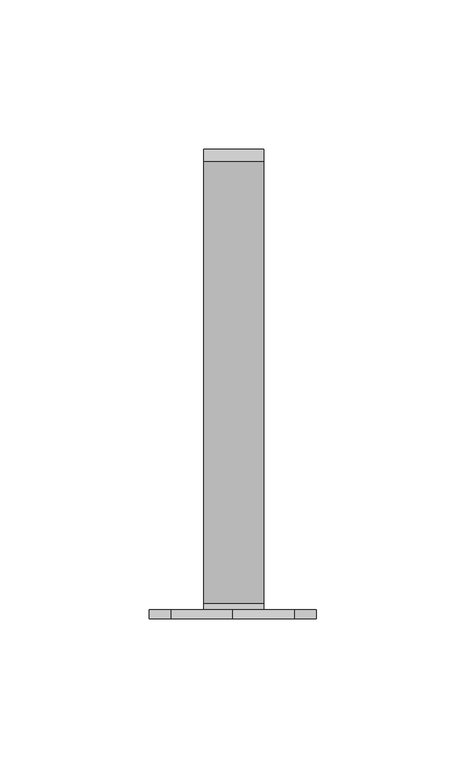
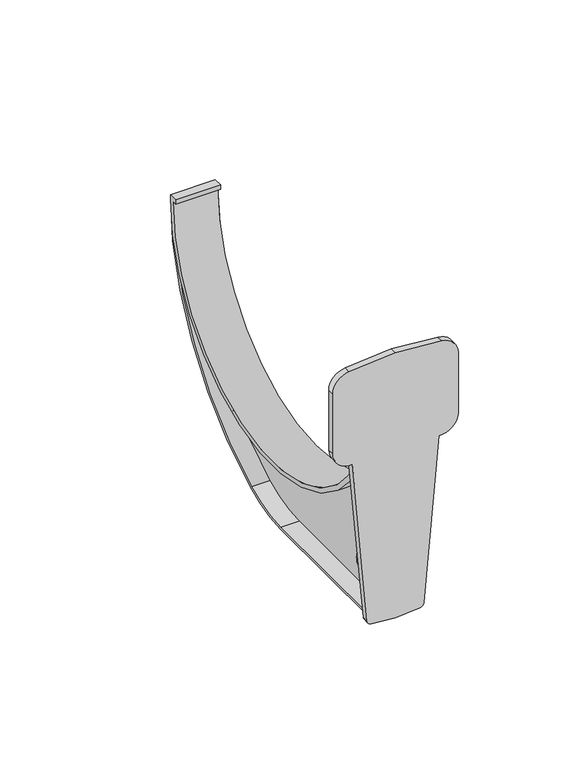
"""IFC4 building model written with IfcOpenShell, lengths in millimetres: proxy geometry, ➾ Кронштейн пластиковый с удлинителем боковым : ➾ Кронштейн пластиковый с удлинителем боковым."""

from ifc_helpers import new_model, si_unit, point, frame, frame_2d, origin, place, context, project, spatial, polyline, circle_curve, trimmed, segment, composite_curve, outline, extrude, source, transform, mapped, element, save
from ifc_brep_helpers import plane_surface, cylinder_surface, revolved_surface, advanced_brep


def generic_models_82e1240d(model_context):
    return source(origin(), model_context, "Body", "SolidModel", [
        advanced_brep(
        [(10.0, 78.1, 0.0), (10.0, 78.1, 2.0), (10.0, 74.055208, 2.0), (10.0, 74.055208, 0.0), (10.0, 76.1, 0.0), (10.0, -76.1, 0.0), (10.0, -76.1, -17.5613211), (-10.0, -76.1, 0.0), (-10.0, 76.1, 0.0), (-10.0, 74.055208, 0.0), (-10.0, 74.055208, 2.0), (-10.0, 78.1, 2.0), (-10.0, 78.1, 0.0), (-10.0, -76.1, -17.5613211), (1.5, -76.1, -17.5613211), (1.5, 71.6158231, -31.1574048), (-1.5, 71.6158231, -31.1574048), (-1.5, -76.1, -17.5613211), (1.5, 76.1, 0.0), (-1.5, 76.1, 0.0), (-1.5, -76.1, 0.0), (1.5, -76.1, 0.0), (1.5, -76.1, -104.0), (1.5, -7.1341862, -104.0), (1.5, 15.3939056, -98.6372612), (1.5, -56.130388, -98.4344464), (1.5, -70.3490278, -98.4344464), (1.5, -70.3490278, -76.8934543), (1.5, -66.9911788, -75.5025877), (1.5, -52.5948541, -89.8989125), (-1.5, 15.3939056, -98.6372612), (-1.5, -7.1341862, -104.0), (-1.5, -76.1, -104.0), (-1.5, -70.3490278, -98.4344464), (-1.5, -56.130388, -98.4344464), (-1.5, -52.5948541, -89.8989125), (-1.5, -66.9911788, -75.5025877), (-1.5, -70.3490278, -76.8934543), (-11.1198282, -79.1, -104.5534176), (-0.2916415, -79.1, -105.5007612), (10.5365453, -79.1, -104.5534176), (12.3546233, -79.1, -102.7353397), (19.0268291, -79.1, -26.4716782), (27.7083585, -79.1, -18.5007612), (27.7083585, -79.1, 9.7189069), (20.4056045, -79.1, 17.6884644), (-0.2807205, -79.1, 19.4982834), (-20.9881575, -79.1, 17.6885282), (-28.2916415, -79.1, 9.7189069), (-28.2916415, -79.1, -18.5007612), (-19.610112, -79.1, -26.4716782), (-12.9379062, -79.1, -102.7353397), (-11.1198282, -76.1, -104.5534176), (-12.9379062, -76.1, -102.7353397), (-19.610112, -76.1, -26.4716782), (-28.2916415, -76.1, -18.5007612), (-28.2916415, -76.1, 9.7189069), (-20.9881575, -76.1, 17.6885283), (-0.2807205, -76.1, 19.4982834), (20.4056045, -76.1, 17.6884644), (27.7083585, -76.1, 9.7189069), (27.7083585, -76.1, -18.5007612), (19.0268291, -76.1, -26.4716782), (12.3546233, -76.1, -102.7353397), (10.5365453, -76.1, -104.5534176), (-0.2916415, -76.1, -105.5007612), (10.0, -76.1, 2.0), (-10.0, -76.1, 2.0), (-10.0, -74.1, 2.0), (10.0, -74.1, 2.0), (-10.0, -74.1, 0.0), (10.0, -74.1, 0.0)],
        [
            (0, 1),
            (1, 2),
            (2, 3),
            (3, 4),
            (4, 5, circle_curve(frame((10.0, 0.0, 0.0), z_axis=(-1.0, 0.0, 0.0), x_axis=(0.0, 1.0, 0.0)), 76.1)),
            (5, 6),
            (6, 0, circle_curve(frame((10.0, 0.0, 0.0), z_axis=(1.0, 0.0, 0.0), x_axis=(0.0, 1.0, 0.0)), 78.1)),
            (7, 8, circle_curve(frame((-10.0, 0.0, 0.0), z_axis=(1.0, 0.0, 0.0), x_axis=(0.0, 1.0, 0.0)), 76.1)),
            (8, 9),
            (9, 10),
            (10, 11),
            (11, 12),
            (12, 13, circle_curve(frame((-10.0, 0.0, 0.0), z_axis=(-1.0, 0.0, 0.0), x_axis=(0.0, 1.0, 0.0)), 78.1)),
            (13, 7),
            (12, 0),
            (6, 14),
            (14, 15, circle_curve(frame((1.5, 0.0, 0.0), z_axis=(1.0, 0.0, 0.0), x_axis=(0.0, 1.0, 0.0)), 78.1)),
            (15, 16),
            (16, 17, circle_curve(frame((-1.5, 0.0, 0.0), z_axis=(-1.0, 0.0, 0.0), x_axis=(0.0, 1.0, 0.0)), 78.1)),
            (17, 13),
            (4, 18),
            (18, 19),
            (19, 8),
            (7, 20),
            (20, 21),
            (21, 5),
            (22, 23),
            (23, 24, circle_curve(frame((1.5, -7.1341862, -54.0), z_axis=(1.0, 0.0, 0.0), x_axis=(0.0, 1.0, 0.0)), 50.0)),
            (24, 15, circle_curve(frame((1.5, -34.3875821, 0.0), z_axis=(1.0, 0.0, 0.0), x_axis=(0.0, 1.0, 0.0)), 110.4875821)),
            (14, 22),
            (25, 26),
            (26, 27),
            (27, 28, circle_curve(frame((1.5, -68.3820454, -76.8934543), z_axis=(-1.0, 0.0, 0.0), x_axis=(0.0, 1.0, 0.0)), 1.9669824)),
            (28, 29),
            (29, 25, circle_curve(frame((1.5, -56.130388, -93.4344464), z_axis=(-1.0, 0.0, 0.0), x_axis=(0.0, 1.0, 0.0)), 5.0)),
            (30, 31, circle_curve(frame((-1.5, -7.1341862, -54.0), z_axis=(-1.0, 0.0, 0.0), x_axis=(0.0, 1.0, 0.0)), 50.0)),
            (31, 32),
            (32, 17),
            (16, 30, circle_curve(frame((-1.5, -34.3875821, 0.0), z_axis=(-1.0, 0.0, 0.0), x_axis=(0.0, 1.0, 0.0)), 110.4875821)),
            (33, 34),
            (34, 35, circle_curve(frame((-1.5, -56.130388, -93.4344464), z_axis=(1.0, 0.0, 0.0), x_axis=(0.0, 1.0, 0.0)), 5.0)),
            (35, 36),
            (36, 37, circle_curve(frame((-1.5, -68.3820454, -76.8934543), z_axis=(1.0, 0.0, 0.0), x_axis=(0.0, 1.0, 0.0)), 1.9669824)),
            (37, 33),
            (22, 32),
            (31, 23),
            (30, 24),
            (38, 39),
            (39, 40),
            (40, 41, circle_curve(frame((10.3622339, -79.1, -102.5610282), z_axis=(0.0, -1.0, 0.0), x_axis=(1.0, 0.0, 0.0)), 2.0)),
            (41, 42),
            (42, 43, circle_curve(frame((19.7083585, -79.1, -18.5007612), z_axis=(0.0, -1.0, 0.0), x_axis=(1.0, 0.0, 0.0)), 8.0)),
            (43, 44),
            (44, 45, circle_curve(frame((19.7083585, -79.1, 9.7189069), z_axis=(0.0, -1.0, 0.0), x_axis=(1.0, 0.0, 0.0)), 8.0)),
            (45, 46),
            (46, 47),
            (47, 48, circle_curve(frame((-20.2916415, -79.1, 9.7189069), z_axis=(0.0, -1.0, 0.0), x_axis=(1.0, 0.0, 0.0)), 8.0)),
            (48, 49),
            (49, 50, circle_curve(frame((-20.2916415, -79.1, -18.5007612), z_axis=(0.0, -1.0, 0.0), x_axis=(1.0, 0.0, 0.0)), 8.0)),
            (50, 51),
            (51, 38, circle_curve(frame((-10.9455168, -79.1, -102.5610282), z_axis=(0.0, -1.0, 0.0), x_axis=(1.0, 0.0, 0.0)), 2.0)),
            (52, 53, circle_curve(frame((-10.9455168, -76.1, -102.5610282), z_axis=(0.0, 1.0, 0.0), x_axis=(1.0, 0.0, 0.0)), 2.0)),
            (53, 54),
            (54, 55, circle_curve(frame((-20.2916415, -76.1, -18.5007612), z_axis=(0.0, 1.0, 0.0), x_axis=(1.0, 0.0, 0.0)), 8.0)),
            (55, 56),
            (56, 57, circle_curve(frame((-20.2916415, -76.1, 9.7189069), z_axis=(0.0, 1.0, 0.0), x_axis=(1.0, 0.0, 0.0)), 8.0)),
            (57, 58),
            (58, 59),
            (59, 60, circle_curve(frame((19.7083585, -76.1, 9.7189069), z_axis=(0.0, 1.0, 0.0), x_axis=(1.0, 0.0, 0.0)), 8.0)),
            (60, 61),
            (61, 62, circle_curve(frame((19.7083585, -76.1, -18.5007612), z_axis=(0.0, 1.0, 0.0), x_axis=(1.0, 0.0, 0.0)), 8.0)),
            (62, 63),
            (63, 64, circle_curve(frame((10.3622339, -76.1, -102.5610282), z_axis=(0.0, 1.0, 0.0), x_axis=(1.0, 0.0, 0.0)), 2.0)),
            (64, 65),
            (65, 52),
            (5, 66),
            (66, 67),
            (67, 7),
            (38, 52),
            (65, 39),
            (64, 40),
            (63, 41),
            (62, 42),
            (61, 43),
            (60, 44),
            (59, 45),
            (58, 46),
            (57, 47),
            (56, 48),
            (55, 49),
            (54, 50),
            (53, 51),
            (33, 26),
            (25, 34),
            (35, 29),
            (28, 36),
            (37, 27),
            (68, 67),
            (66, 69),
            (69, 68),
            (70, 71),
            (71, 5),
            (7, 70),
            (68, 70),
            (71, 69),
            (11, 1),
            (10, 2),
            (9, 3),
        ],
        [
            plane_surface(frame((10.0, -76.1, 0.0), z_axis=(1.0, 0.0, 0.0), x_axis=(0.0, -1.0, 0.0))),
            plane_surface(frame((-10.0, -76.1, 0.0), z_axis=(-1.0, 0.0, 0.0), x_axis=(0.0, 1.0, 0.0))),
            cylinder_surface(frame((-10.0, 0.0, 0.0), z_axis=(1.0, 0.0, 0.0), x_axis=(0.0, 1.0, 0.0)), 78.1),
            revolved_surface(polyline([(-10.0, 76.1, 0.0), (10.0, 76.1, 0.0)]), (-10.0, 0.0, 0.0), (-1.0, 0.0, 0.0)),
            plane_surface(frame((1.5, 76.1, 0.0), z_axis=(1.0, 0.0, 0.0), x_axis=(0.0, 0.0, -1.0))),
            plane_surface(frame((-1.5, 76.1, 0.0), z_axis=(-1.0, 0.0, 0.0), x_axis=(0.0, 0.0, 1.0))),
            plane_surface(frame((1.5, -76.1, -104.0), z_axis=(0.0, 0.0, -1.0), x_axis=(-1.0, 0.0, 0.0))),
            cylinder_surface(frame((-1.5, -7.1341862, -54.0), z_axis=(1.0, 0.0, 0.0), x_axis=(0.0, 1.0, 0.0)), 50.0),
            cylinder_surface(frame((-1.5, -34.3875821, 0.0), z_axis=(1.0, 0.0, 0.0), x_axis=(0.0, 1.0, 0.0)), 110.4875821),
            plane_surface(frame((-11.1198282, -79.1, -104.5534176), z_axis=(0.0, -1.0000000000000002, 0.0), x_axis=(0.9961946980917458, 0.0, -0.08715574274765676))),
            plane_surface(frame((-11.1198282, -76.1, -104.5534176), z_axis=(0.0, 1.0000000000000002, 0.0), x_axis=(-0.9961946980917458, 0.0, 0.08715574274765676))),
            plane_surface(frame((-11.1198282, -79.1, -104.5534176), z_axis=(-0.08715574274765676, 0.0, -0.9961946980917458), x_axis=(0.0, 1.0, 0.0))),
            plane_surface(frame((-0.2916415, -79.1, -105.5007612), z_axis=(0.0871557427476553, 0.0, -0.9961946980917459), x_axis=(0.0, 1.0, 0.0))),
            cylinder_surface(frame((10.3622339, -76.1, -102.5610282), z_axis=(0.0, -1.0, 0.0), x_axis=(1.0, 0.0, 0.0)), 2.0),
            plane_surface(frame((12.3546233, -79.1, -102.7353397), z_axis=(0.9961946980917455, 0.0, -0.08715574274765876), x_axis=(0.0, 1.0, 0.0))),
            cylinder_surface(frame((19.7083585, -76.1, -18.5007612), z_axis=(0.0, -1.0, 0.0), x_axis=(1.0, 0.0, 0.0)), 8.0),
            plane_surface(frame((27.7083585, -79.1, -18.5007612), z_axis=(1.0, 0.0, 0.0), x_axis=(0.0, 1.0, 0.0))),
            cylinder_surface(frame((19.7083585, -76.1, 9.7189069), z_axis=(0.0, -1.0, 0.0), x_axis=(1.0, 0.0, 0.0)), 8.0),
            plane_surface(frame((20.4056045, -79.1, 17.6884644), z_axis=(0.08715574274766355, 0.0, 0.9961946980917451), x_axis=(0.0, 1.0, 0.0))),
            plane_surface(frame((-0.2807205, -79.1, 19.4982834), z_axis=(-0.08706451221038128, 0.0, 0.9962026755201817), x_axis=(0.0, 1.0, 0.0))),
            cylinder_surface(frame((-20.2916415, -76.1, 9.7189069), z_axis=(0.0, -1.0, 0.0), x_axis=(1.0, 0.0, 0.0)), 8.0),
            plane_surface(frame((-28.2916415, -79.1, 9.7189069), z_axis=(-1.0, 0.0, 0.0), x_axis=(0.0, 1.0, 0.0))),
            cylinder_surface(frame((-20.2916415, -76.1, -18.5007612), z_axis=(0.0, -1.0, 0.0), x_axis=(1.0, 0.0, 0.0)), 8.0),
            plane_surface(frame((-19.610112, -79.1, -26.4716782), z_axis=(-0.9961946980917457, 0.0, -0.08715574274765732), x_axis=(0.0, 1.0, 0.0))),
            cylinder_surface(frame((-10.9455168, -76.1, -102.5610282), z_axis=(0.0, -1.0, 0.0), x_axis=(1.0, 0.0, 0.0)), 2.0),
            plane_surface(frame((10.0, -70.3490278, -98.4344464), z_axis=(0.0, 0.0, 1.0), x_axis=(-1.0, 0.0, 0.0))),
            plane_surface(frame((10.0, -52.5948541, -89.8989125), z_axis=(0.0, -0.7071067811865492, -0.7071067811865459), x_axis=(-1.0, 0.0, 0.0))),
            plane_surface(frame((10.0, -70.3490278, -76.8934543), z_axis=(0.0, 1.0, 0.0), x_axis=(-1.0, 0.0, 0.0))),
            revolved_surface(polyline([(1.5, -51.130388, -93.4344464), (-1.5, -51.130388, -93.4344464)]), (-10.0, -56.130388, -93.4344464), (1.0, 0.0, 0.0)),
            revolved_surface(polyline([(1.5, -66.41506299999999, -76.8934543), (-1.5, -66.41506299999999, -76.8934543)]), (-10.0, -68.3820454, -76.8934543), (1.0, 0.0, 0.0)),
            plane_surface(frame((-10.0, -76.1, 2.0), z_axis=(0.0, 0.0, 1.0), x_axis=(0.0, -1.0, 0.0))),
            plane_surface(frame((-10.0, -76.1, 0.0), z_axis=(0.0, 0.0, -1.0), x_axis=(0.0, 1.0, 0.0))),
            plane_surface(frame((-10.0, -74.1, 2.0), z_axis=(-1.0, 0.0, 0.0), x_axis=(0.0, 0.0, -1.0))),
            plane_surface(frame((10.0, -76.1, 2.0), z_axis=(1.0, 0.0, 0.0), x_axis=(0.0, 0.0, -1.0))),
            plane_surface(frame((10.0, -74.1, 2.0), z_axis=(0.0, 1.0, 0.0), x_axis=(0.0, 0.0, -1.0))),
            plane_surface(frame((10.0, 78.1, 0.0), z_axis=(0.0, 1.0, 0.0), x_axis=(-1.0, 0.0, 0.0))),
            plane_surface(frame((10.0, 78.1, 2.0), z_axis=(0.0, 0.0, 1.0), x_axis=(-1.0, 0.0, 0.0))),
            plane_surface(frame((10.0, 74.055208, 2.0), z_axis=(0.0, -1.0, 0.0), x_axis=(-1.0, 0.0, 0.0))),
            plane_surface(frame((10.0, 74.055208, 0.0), z_axis=(0.0, 0.0, -1.0), x_axis=(-1.0, 0.0, 0.0))),
        ],
        [
            (0, [[1, 2, 3, 4, 5, 6, 7]]),
            (1, [[8, 9, 10, 11, 12, 13, 14]]),
            (2, [[15, -7, 16, 17, 18, 19, 20, -13]]),
            (3, [[-5, 21, 22, 23, -8, 24, 25, 26]]),
            (4, [[27, 28, 29, -17, 30], [31, 32, 33, 34, 35]]),
            (5, [[36, 37, 38, -19, 39], [40, 41, 42, 43, 44]]),
            (6, [[-27, 45, -37, 46]]),
            (7, [[-28, -46, -36, 47]]),
            (8, [[-47, -39, -18, -29]]),
            (9, [[48, 49, 50, 51, 52, 53, 54, 55, 56, 57, 58, 59, 60, 61]]),
            (10, [[62, 63, 64, 65, 66, 67, 68, 69, 70, 71, 72, 73, 74, 75], [-6, 76, 77, 78, -14, -20, -38, -45, -30, -16]]),
            (11, [[-48, 79, -75, 80]]),
            (12, [[-49, -80, -74, 81]]),
            (13, [[-50, -81, -73, 82]]),
            (14, [[-51, -82, -72, 83]]),
            (15, [[-52, -83, -71, 84]]),
            (16, [[-53, -84, -70, 85]]),
            (17, [[-54, -85, -69, 86]]),
            (18, [[-55, -86, -68, 87]]),
            (19, [[-56, -87, -67, 88]]),
            (20, [[-57, -88, -66, 89]]),
            (21, [[-58, -89, -65, 90]]),
            (22, [[-59, -90, -64, 91]]),
            (23, [[-60, -91, -63, 92]]),
            (24, [[-61, -92, -62, -79]]),
            (25, [[93, -31, 94, -40]]),
            (26, [[95, -34, 96, -42]]),
            (27, [[-93, -44, 97, -32]]),
            (28, [[-95, -41, -94, -35]]),
            (29, [[-97, -43, -96, -33]]),
            (30, [[98, -77, 99, 100]]),
            (31, [[101, 102, -26, -25, -24, 103]]),
            (32, [[-98, 104, -103, -78]]),
            (33, [[-99, -76, -102, 105]]),
            (34, [[-100, -105, -101, -104]]),
            (35, [[-1, -15, -12, 106]]),
            (36, [[-2, -106, -11, 107]]),
            (37, [[-3, -107, -10, 108]]),
            (38, [[-4, -108, -9, -23, -22, -21]]),
        ],
    ),
        extrude(outline(composite_curve([segment(trimmed(circle_curve(frame_2d((-7.1341862, -53.026974)), 50.0), [point((-7.1341862, -103.026974))], [point((15.3939056, -97.6642352))], True, "CARTESIAN"), True, "CONTINUOUS"), segment(trimmed(circle_curve(frame_2d((-34.3875821, 0.973026)), 110.4875821), [point((15.3939056, -97.6642352))], [point((76.0957154, 0.0))], True, "CARTESIAN"), True, "CONTINUOUS"), segment(polyline([(76.0957154, 0.0), (74.055208, 0.0), (74.055208, 2.0), (78.1, 2.0)]), True, "CONTINUOUS"), segment(trimmed(circle_curve(frame_2d((-34.3875821, 2.0)), 112.4875821), [point((78.1, 2.0))], [point((16.2950292, -98.4227516))], False, "CARTESIAN"), True, "CONTINUOUS"), segment(trimmed(circle_curve(frame_2d((-7.1341862, -52.0)), 52.0), [point((16.2950292, -98.4227516))], [point((-7.1341862, -104.0))], False, "CARTESIAN"), True, "CONTINUOUS"), segment(polyline([(-7.1341862, -104.0), (-76.1, -104.0), (-76.1, -103.026974), (-7.1341862, -103.026974)]), True, "CONTINUOUS")], self_intersect=False)), frame((-10.0, 0.0, 0.0), z_axis=(1.0, 0.0, 0.0), x_axis=(0.0, 1.0, 0.0)), (0.0, 0.0, 1.0), 20.0),
    ])


if __name__ == "__main__":
    model = new_model("IFC4")
    model_context = context("Model", 3, world=origin())
    ifc_project = project(units=[si_unit("LENGTHUNIT", "METRE", prefix="MILLI")], contexts=[model_context])
    site = spatial("IfcSite", under=ifc_project)
    building = spatial("IfcBuilding", under=site)
    placement = place(None, origin())
    generic_models_shape = generic_models_82e1240d(model_context)
    element("IfcBuildingElementProxy", 1, Name="➾ Кронштейн пластиковый с удлинителем боковым : ➾ Кронштейн пластиковый с удлинителем боковым", ObjectType="➾ Кронштейн пластиковый с удлинителем боковым : ➾ Кронштейн пластиковый с удлинителем боковым", at=placement, inside=building, context=model_context, shape_type="MappedRepresentation", body=[
        mapped(generic_models_shape, transform((0.0, 0.0, 0.0), x_axis=(1.0, 0.0, 0.0), y_axis=(0.0, 1.0, 0.0), z_axis=(0.0, 0.0, 1.0))),
    ])
    save(model, "model.ifc")

# Revit data of these elements
# Type "➾ Кронштейн пластиковый с удлинителем боковым : ➾ Кронштейн пластиковый с удлинителем боковым"
#   Description = "Используется для монтажа желоба на\r\nкарнизе кровли. Крепится к лобовой\r\nдоске"
#   Manufacturer = "ТехноНИКОЛЬ"
#   Model = "Комплектующие к водосточным системам"
#   URL = "https://tn-vodostok.ru/catalog/pvh/"
#   ADSK_Обозначение = "ТехноНИКОЛЬ"
#   ADSK_Наименование краткое = "Кронштейн"
#   ADSK_Наименование = "Кронштейн пластиковый"
#   ADSK_Масса_Текст = ""
#   ADSK_Марка = ""
#   ADSK_Код изделия = ""
#   ADSK_Завод-изготовитель = "ТехноНИКОЛЬ"
#   ADSK_Единица измерения = "шт."
#   ADSK_Группирование = "Комплектующие к водосточным системам"
#   ADSK_URL страницы изделия = "https://tn-vodostok.ru/catalog/pvh/"
#   ADSK_URL документации изделия = "https://tn-vodostok.ru/upload/iblock/c42/c427963cb77eb5c3c51f0cfb870e9e52.pdf"
#   Угол поворота кронштейна [instance default] = 20.00°
#   Длина пластины [instance default] = 200 mm
#   ADSK_Размер_Ширина = 20 mm
#   ADSK_Размер_Высота = 125 mm
#   ADSK_Количество = 1
#   Видимость [instance default] = yes
#   ADSK_Материал [instance default] = TN_Пластик_Коричневый_RAL8019
#   Default Elevation = 0
# Element 1 (IfcBuildingElementProxy, "➾ Кронштейн пластиковый с удлинителем боковым : ➾ Кронштейн пластиковый с удлинителем боковым")
#   Угол поворота кронштейна = 45.00°
#   Materials on its faces: "TN_Пластик_Коричневый_RAL8019"
# Materials
#   "TN_Пластик_Коричневый_RAL8019": class "Типовые", colour RGB 61 54 53, transparency 0, Cost = 0
